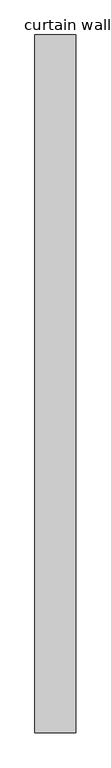
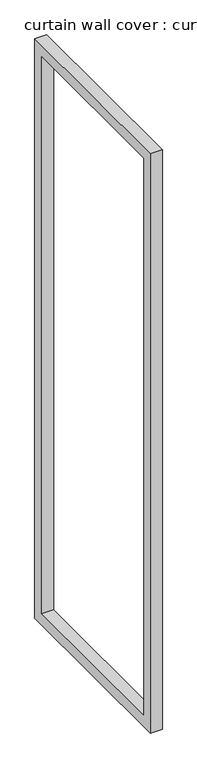
"""IFC4 building model written with IfcOpenShell, lengths in millimetres: proxy geometry, curtain wall cover : curtain wall cover."""

from ifc_helpers import new_model, si_unit, frame, origin, place, context, project, spatial, polyline, outline, extrude, source, transform, mapped, element, save


def curtain_wall_cover_curtain_wall_cover_1924c590(model_context):
    return source(origin(), model_context, "Body", "SweptSolid", [
        extrude(outline(polyline([(-531.6073833, 9196.8), (-531.6073833, 3998.4), (-2234.8073833, 3998.4), (-2234.8073833, 9196.8), (-531.6073833, 9196.8)]), holes=[polyline([(-2133.2073833, 9095.2), (-2133.2073833, 4100.0), (-633.2073833, 4100.0), (-633.2073833, 9095.2), (-2133.2073833, 9095.2)])]), frame((16099.9, 0.0, 0.0), z_axis=(1.0, 0.0, 0.0), x_axis=(0.0, 1.0, 0.0)), (0.0, 0.0, 1.0), 100.0),
    ])


if __name__ == "__main__":
    model = new_model("IFC4")
    model_context = context("Model", 3, world=origin())
    ifc_project = project(units=[si_unit("LENGTHUNIT", "METRE", prefix="MILLI")], contexts=[model_context])
    site = spatial("IfcSite", under=ifc_project)
    building = spatial("IfcBuilding", under=site)
    placement = place(None, origin())
    curtain_wall_cover_curtain_wall_cover_shape = curtain_wall_cover_curtain_wall_cover_1924c590(model_context)
    element("IfcBuildingElementProxy", 1, Name="curtain wall cover : curtain wall cover", ObjectType="curtain wall cover : curtain wall cover", at=placement, inside=building, context=model_context, shape_type="MappedRepresentation", body=[
        mapped(curtain_wall_cover_curtain_wall_cover_shape, transform((0.0, 0.0, 0.0), x_axis=(1.0, 0.0, 0.0), y_axis=(0.0, 1.0, 0.0), z_axis=(0.0, 0.0, 1.0))),
    ])
    save(model, "model.ifc")

# Revit data of these elements
# Element 1 (IfcBuildingElementProxy, "curtain wall cover : curtain wall cover")
#   Materials on its faces: "wooden-3"
# Materials
#   "wooden-3": class "Generic", colour RGB 120 120 120, transparency 0, Cost = 0
